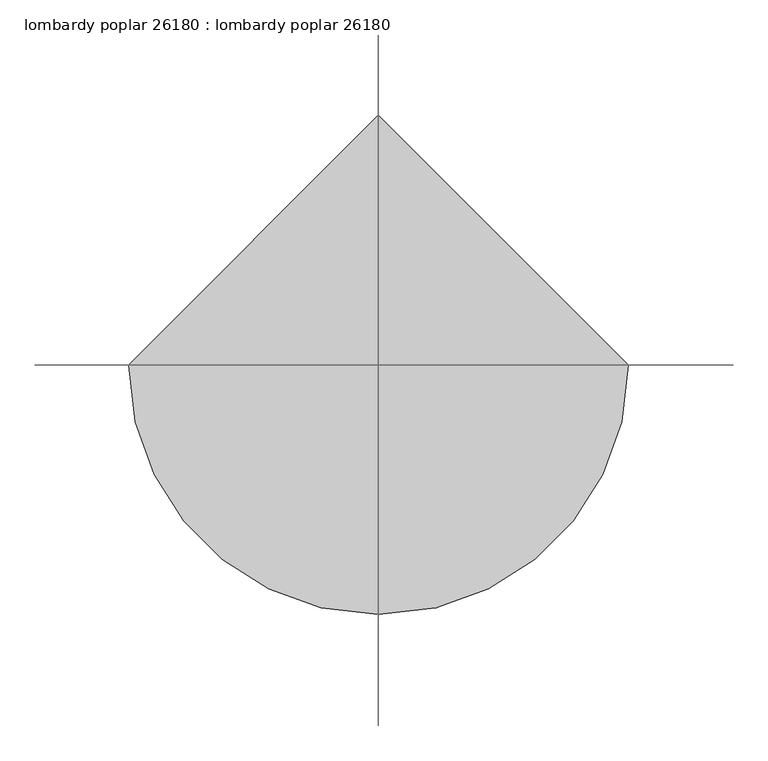
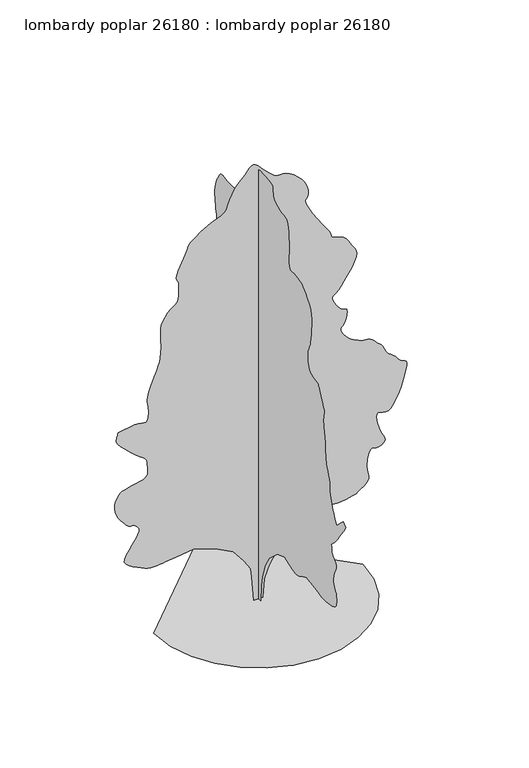
"""IFC4 building model written with IfcOpenShell, lengths in millimetres: proxy geometry, lombardy poplar 26180 : lombardy poplar 26180."""

from ifc_helpers import new_model, si_unit, origin, place, context, project, spatial, triangles, source, transform, mapped, element, save


def lombardy_poplar_26180_lombardy_poplar_26180_01077960(model_context):
    return source(origin(), model_context, "Body", "Tessellation", [
        triangles([(0.0009695, 113.8156909, 0.0), (0.0009695, -104.8345258, 0.0), (0.0009695, -123.055434, 437.3009239), (0.0009695, -177.7179314, 728.8340738), (0.0009695, -323.483707, 1129.6911467), (0.0009695, -505.6928613, 1439.4461494), (0.0009695, -870.1086628, 1767.420607), (0.0009695, -1216.3049732, 1894.9664555), (0.0009695, -1398.5142002, 1822.0838402), (0.0009695, -1476.390406, 1795.1523445), (0.0009695, -1552.9941605, 1770.6083485), (0.0009695, -1627.0451637, 1750.8472), (0.0009695, -1697.2735806, 1738.2588696), (0.0009695, -1762.3991112, 1735.2286766), (0.0009695, -1821.1516296, 1744.1542946), (0.0009695, -1872.2563591, 1767.420607), (0.0009695, -1919.1091679, 1797.0624023), (0.0009695, -1965.9644474, 1823.8364948), (0.0009695, -2012.8172562, 1848.2204716), (0.0009695, -2059.6700649, 1870.6891582), (0.0009695, -2106.5227283, 1891.7279903), (0.0009695, -2153.3780079, 1911.8067066), (0.0009695, -2200.2308167, 1931.4103065), (0.0009695, -2582.8711235, 1876.7470734), (0.0009695, -2649.2156204, 1861.2353748), (0.0009695, -2715.4080917, 1846.3611374), (0.0009695, -2781.27006, 1832.7619675), (0.0009695, -2846.6750793, 1821.0754715), (0.0009695, -2911.4196739, 1811.9366398), (0.0009695, -2975.3765259, 1805.987875), (0.0009695, -3038.3939003, 1803.8619873), (0.0009695, -3111.6472778, 1806.252103), (0.0009695, -3200.5217949, 1814.0625275), (0.0009695, -3296.0764275, 1828.2459641), (0.0009695, -3389.4213112, 1849.7596218), (0.0009695, -3471.5901329, 1879.5614365), (0.0009695, -3533.6930283, 1918.6062916), (0.0009695, -3566.7892639, 1967.8516869), (0.0009695, -3579.2353065, 2021.4507408), (0.0009695, -3585.9154221, 2073.1371208), (0.0009695, -3587.8205383, 2123.2333363), (0.0009695, -3585.9154221, 2172.0521587), (0.0009695, -3581.1401321, 2219.915807), (0.0009695, -3574.4347275, 2267.139378), (0.0009695, -3566.7892639, 2314.0455265), (0.0009695, -3532.0422569, 2353.5170998), (0.0009695, -3499.7078934, 2395.5361919), (0.0009695, -3472.1235306, 2442.6555542), (0.0009695, -3451.7273918, 2497.4231415), (0.0009695, -3440.907122, 2562.3988266), (0.0009695, -3441.9992065, 2640.0972816), (0.0009695, -3457.4677391, 2733.1372421), (0.0009695, -3484.5187042, 2825.1865654), (0.0009695, -3515.3799019, 2900.6752716), (0.0009695, -3544.9708282, 2963.0830902), (0.0009695, -3568.1862717, 3015.940329), (0.0009695, -3579.9210205, 3062.7525879), (0.0009695, -3575.0695724, 3106.9993057), (0.0009695, -3548.5775848, 3152.2110809), (0.0009695, -3509.7918709, 3193.1050964), (0.0009695, -3472.6063499, 3225.0836678), (0.0009695, -3438.6212151, 3252.6171616), (0.0009695, -3409.3857903, 3280.1253662), (0.0009695, -3386.5511375, 3312.1039375), (0.0009695, -3371.6668716, 3352.997953), (0.0009695, -3366.3581841, 3407.3030685), (0.0009695, -3362.7005585, 3460.5158089), (0.0009695, -3354.9027786, 3498.4634926), (0.0009695, -3347.7145546, 3525.8699593), (0.0009695, -3345.9620453, 3547.5360786), (0.0009695, -3354.4202499, 3568.2624298), (0.0009695, -3377.8388786, 3592.7987228), (0.0009695, -3421.0188011, 3625.9458275), (0.0009695, -3481.5215034, 3679.8698616), (0.0009695, -3552.5654228, 3760.5655174), (0.0009695, -3632.3465996, 3863.5624283), (0.0009695, -3719.1381042, 3984.4155167), (0.0009695, -3811.2130074, 4118.6541252), (0.0009695, -3906.7676399, 4261.8084686), (0.0009695, -4004.1003616, 4409.432888), (0.0009695, -3894.7788368, 4518.779702), (0.0009695, -3749.0086647, 4391.221209), (0.0009695, -3603.2382019, 4227.2390671), (0.0009695, -3579.7434151, 4258.785688), (0.0009695, -3555.9689941, 4292.2630051), (0.0009695, -3531.5088593, 4329.5499733), (0.0009695, -3506.1342453, 4372.5775795), (0.0009695, -3479.4643616, 4423.2506493), (0.0009695, -3451.1939941, 4483.4992973), (0.0009695, -3421.0188011, 4555.2033508), (0.0009695, -3390.0055779, 4628.5837555), (0.0009695, -3360.2623352, 4695.8683113), (0.0009695, -3333.0587631, 4762.2383881), (0.0009695, -3309.6910034, 4832.7233299), (0.0009695, -3291.4028755, 4912.4536377), (0.0009695, -3279.5158104, 5006.5351044), (0.0009695, -3275.248629, 5120.0473618), (0.0009695, -3267.0697678, 5234.8554703), (0.0009695, -3245.5050957, 5333.3820145), (0.0009695, -3215.0252701, 5421.7481323), (0.0009695, -3180.0747871, 5505.9238083), (0.0009695, -3145.0993057, 5592.0551788), (0.0009695, -3114.6191895, 5686.1110657), (0.0009695, -3093.0545174, 5794.238768), (0.0009695, -3079.5672592, 5892.1298859), (0.0009695, -3069.8899429, 5959.4403122), (0.0009695, -3063.4130127, 6007.9286316), (0.0009695, -3059.4760437, 6049.4319122), (0.0009695, -3057.4691895, 6095.6854843), (0.0009695, -3056.7073174, 6158.5246719), (0.0009695, -3056.6055794, 6249.735965), (0.0009695, -3052.5671631, 6343.1320084), (0.0009695, -3042.1532639, 6412.2958099), (0.0009695, -3027.9291321, 6468.709227), (0.0009695, -3012.4097305, 6523.8523727), (0.0009695, -2998.1858894, 6589.2065231), (0.0009695, -2987.7716995, 6676.2017944), (0.0009695, -2983.7332832, 6796.3688782), (0.0009695, -2989.2957344, 6908.7381821), (0.0009695, -3001.5638809, 6976.78461), (0.0009695, -3013.8576073, 7018.6948425), (0.0009695, -3019.4200584, 7052.6288177), (0.0009695, -3011.6222786, 7096.7737976), (0.0009695, -2983.7332832, 7169.2908829), (0.0009695, -2929.0723755, 7288.340593), (0.0009695, -2866.7410057, 7418.1088348), (0.0009695, -2818.7857933, 7514.4256302), (0.0009695, -2782.7688057, 7582.8528488), (0.0009695, -2756.3021072, 7628.9541046), (0.0009695, -2737.0233421, 7658.3418457), (0.0009695, -2722.5201576, 7676.5535248), (0.0009695, -2710.4043274, 7689.2027527), (0.0009695, -2636.5666832, 7701.2421341), (0.0009695, -2564.8117607, 7715.3901077), (0.0009695, -2497.1818771, 7733.6523651), (0.0009695, -2435.7748695, 7758.1380798), (0.0009695, -2382.6507866, 7790.9296829), (0.0009695, -2339.8900246, 7834.0584457), (0.0009695, -2309.5548122, 7889.6335419), (0.0009695, -2289.3160767, 7951.0257248), (0.0009695, -2274.8152176, 8010.5377899), (0.0009695, -2265.0921192, 8068.4243729), (0.0009695, -2259.1968395, 8125.0662643), (0.0009695, -2256.1691174, 8180.7425171), (0.0009695, -2255.0515984, 8235.7589264), (0.0009695, -2254.8940498, 8290.4707031), (0.0009695, -2285.970932, 8345.7405853), (0.0009695, -2316.0901691, 8404.491069), (0.0009695, -2344.2968777, 8470.25159), (0.0009695, -2369.6358833, 8546.5277481), (0.0009695, -2391.1521572, 8636.8495605), (0.0009695, -2407.8857288, 8744.6726303), (0.0009695, -2418.8812786, 8873.551973), (0.0009695, -2430.0903328, 9004.9206985), (0.0009695, -2443.8493767, 9121.3031296), (0.0009695, -2453.7833633, 9227.8303482), (0.0009695, -2453.5168098, 9329.5572784), (0.0009695, -2436.6765587, 9431.5888412), (0.0009695, -2396.8874176, 9539.0561188), (0.0009695, -2327.7766651, 9657.0390335), (0.0009695, -2247.8811058, 9768.2398041), (0.0009695, -2177.228587, 9854.8798645), (0.0009695, -2111.6764835, 9921.4269653), (0.0009695, -2047.0792637, 9972.3796692), (0.0009695, -1979.2969185, 10012.156311), (0.0009695, -1904.1815907, 10045.2519653), (0.0009695, -1817.5931259, 10076.1128723), (0.0009695, -1725.5334835, 10094.8326599), (0.0009695, -1638.891679, 10096.3058258), (0.0009695, -1560.8554539, 10092.3688568), (0.0009695, -1494.6124043, 10094.8326599), (0.0009695, -1443.3501263, 10115.4325653), (0.0009695, -1410.2540359, 10166.0038971), (0.0009695, -1398.5142002, 10258.3319824), (0.0009695, -1400.4267288, 10362.6756134), (0.0009695, -1404.8895378, 10448.1971375), (0.0009695, -1409.9898079, 10525.1087219), (0.0009695, -1413.8125397, 10603.619046), (0.0009695, -1414.4501461, 10693.9414398), (0.0009695, -1409.9898079, 10806.2345856), (0.0009695, -1398.5142002, 10950.7350677), (0.0009695, -1382.6849339, 11097.4458801), (0.0009695, -1365.5779839, 11211.9737732), (0.0009695, -1345.9235149, 11297.8255096), (0.0009695, -1322.4438435, 11358.4811096), (0.0009695, -1293.8637566, 11397.4694275), (0.0009695, -1258.9083321, 11418.297226), (0.0009695, -1216.3049732, 11424.470105), (0.0009695, -1155.4822323, 11429.9813965), (0.0009695, -1073.3006933, 11446.3641174), (0.0009695, -979.6484882, 11473.2380585), (0.0009695, -884.3986336, 11510.3218414), (0.0009695, -797.4393339, 11557.2608368), (0.0009695, -728.6460766, 11613.8015717), (0.0009695, -687.9020519, 11679.5615112), (0.0009695, -672.8677952, 11749.3607391), (0.0009695, -668.0341513, 11816.289212), (0.0009695, -663.5180752, 11877.4785004), (0.0009695, -649.4413908, 11930.0811035), (0.0009695, -615.9210531, 11971.2041748), (0.0009695, -553.0790314, 11997.9757965), (0.0009695, -451.0296281, 12007.5263763), (0.0009695, -327.7864603, 12011.2087097), (0.0009695, -210.2816959, 12019.0070709), (0.0009695, -102.0189364, 12026.1694244), (0.0009695, -6.5056406, 12027.9216431), (0.0009695, 72.7523407, 12019.4895996), (0.0009695, 132.2489498, 11996.0700989), (0.0009695, 168.4781792, 11952.8657593), (0.0009695, 190.2581361, 11903.7920105), (0.0009695, 211.0820467, 11861.400412), (0.0009695, 234.4553475, 11819.0076508), (0.0009695, 263.8852554, 11769.9094849), (0.0009695, 302.8767344, 11707.4505066), (0.0009695, 354.9364746, 11624.9008942), (0.0009695, 423.5697126, 11515.57966), (0.0009695, 499.5867296, 11399.1204895), (0.0009695, 572.09851, 11297.9778259), (0.0009695, 642.0601553, 11209.5867096), (0.0009695, 710.4292379, 11131.3798553), (0.0009695, 778.1582434, 11060.8446259), (0.0009695, 846.2072874, 10995.3881561), (0.0009695, 915.531399, 10932.4978088), (0.0009695, 983.7404623, 10880.5556305), (0.0009695, 1048.444289, 10847.0786041), (0.0009695, 1110.5954372, 10828.282077), (0.0009695, 1171.1565662, 10820.3069824), (0.0009695, 1231.077618, 10819.3407623), (0.0009695, 1291.3160923, 10821.5766724), (0.0009695, 1352.8322502, 10823.1765747), (0.0009695, 1419.1287849, 10828.7646057), (0.0009695, 1490.5254444, 10841.0324615), (0.0009695, 1563.194846, 10853.3014801), (0.0009695, 1633.3164379, 10858.8639313), (0.0009695, 1697.0626923, 10851.0655701), (0.0009695, 1750.6084064, 10823.1765747), (0.0009695, 1790.1333195, 10768.5159576), (0.0009695, 1824.1844387, 10700.9526398), (0.0009695, 1861.7408672, 10636.2333344), (0.0009695, 1899.617189, 10570.5745514), (0.0009695, 1934.6234825, 10500.1404785), (0.0009695, 1963.5743317, 10421.0953033), (0.0009695, 1983.2847565, 10329.6299561), (0.0009695, 1990.5617832, 10221.8830444), (0.0009695, 1988.4357502, 10111.0130676), (0.0009695, 1982.4871307, 10010.9877777), (0.0009695, 1973.3507698, 9919.2433777), (0.0009695, 1961.6642738, 9833.2381622), (0.0009695, 1948.0651039, 9750.4350769), (0.0009695, 1933.1908665, 9668.2656738), (0.0009695, 1917.6791679, 9584.1667374), (0.0009695, 1914.3314072, 9505.3761978), (0.0009695, 1931.0649788, 9438.0663528), (0.0009695, 1961.1842159, 9378.0967575), (0.0009695, 1997.9989746, 9321.3025497), (0.0009695, 2034.813588, 9263.5682831), (0.0009695, 2064.9328251, 9200.7290955), (0.0009695, 2081.6663967, 9128.6439606), (0.0009695, 2081.1888096, 9058.6668365), (0.0009695, 2066.6854797, 9001.7964706), (0.0009695, 2041.9840805, 8953.1808334), (0.0009695, 2010.9071983, 8908.0707962), (0.0009695, 1977.2826519, 8861.6904877), (0.0009695, 1944.9307022, 8809.2646179), (0.0009695, 1917.6791679, 8745.9934799), (0.0009695, 1901.8472855, 8673.7048691), (0.0009695, 1900.361475, 8598.2164536), (0.0009695, 1911.9412914, 8520.8229218), (0.0009695, 1935.3142834, 8442.7939636), (0.0009695, 1969.2055286, 8365.374852), (0.0009695, 2012.3422852, 8289.8864365), (0.0009695, 2063.4443985, 8217.5978256), (0.0009695, 2116.1951031, 8158.060762), (0.0009695, 2166.3955273, 8113.7884644), (0.0009695, 2215.9584904, 8075.6123062), (0.0009695, 2266.796521, 8034.2101822), (0.0009695, 2320.8222931, 7980.4134659), (0.0009695, 2379.9457191, 7904.924469), (0.0009695, 2446.0820892, 7798.5239868), (0.0009695, 2515.4595406, 7684.1478287), (0.0009695, 2583.8870499, 7588.5931961), (0.0009695, 2652.6194824, 7508.3039108), (0.0009695, 2722.9518173, 7439.8511124), (0.0009695, 2796.1546165, 7379.653624), (0.0009695, 2873.4972794, 7324.2558426), (0.0009695, 2956.2759476, 7270.103334), (0.0009695, 3039.9940933, 7227.3042023), (0.0009695, 3119.5720848, 7202.0063278), (0.0009695, 3195.3148453, 7185.0137604), (0.0009695, 3267.5522964, 7167.0555542), (0.0009695, 3336.6149414, 7138.9125046), (0.0009695, 3402.807122, 7091.3130844), (0.0009695, 3466.4593414, 7015.0113464), (0.0009695, 3525.2604034, 6921.5903046), (0.0009695, 3575.4506538, 6829.7441666), (0.0009695, 3615.1508469, 6741.0728348), (0.0009695, 3642.3797081, 6657.2023727), (0.0009695, 3655.3082794, 6579.6815231), (0.0009695, 3651.9552864, 6510.1619293), (0.0009695, 3630.4414833, 6450.1673355), (0.0009695, 3590.004998, 6392.5348068), (0.0009695, 3534.6075073, 6330.4316208), (0.0009695, 3469.3295151, 6266.1192673), (0.0009695, 3399.2512344, 6201.7813339), (0.0009695, 3329.5028755, 6139.6781479), (0.0009695, 3265.1646515, 6082.0456192), (0.0009695, 3211.3676445, 6031.0934967), (0.0009695, 3161.7869499, 5985.0939789), (0.0009695, 3109.3613708, 5939.7298874), (0.0009695, 3057.8758507, 5893.4001572), (0.0009695, 3011.1906189, 5844.5304657), (0.0009695, 2973.1159081, 5791.5209106), (0.0009695, 2947.4366615, 5732.7710083), (0.0009695, 2938.0386887, 5666.680275), (0.0009695, 2934.1778778, 5597.4141541), (0.0009695, 2924.8816429, 5529.7235184), (0.0009695, 2913.6547119, 5463.0235199), (0.0009695, 2904.0535538, 5396.6025742), (0.0009695, 2899.5323181, 5329.8764145), (0.0009695, 2903.6218941, 5262.2113586), (0.0009695, 2919.8270096, 5192.9452377), (0.0009695, 2944.8458313, 5126.3719757), (0.0009695, 2972.7351173, 5066.5046997), (0.0009695, 3003.0117577, 5012.2248734), (0.0009695, 3035.1935143, 4962.3901245), (0.0009695, 3068.8231476, 4915.908078), (0.0009695, 3103.4178383, 4871.6613602), (0.0009695, 3138.4697685, 4828.5323067), (0.0009695, 3181.1415825, 4835.3141602), (0.0009695, 3222.035598, 4836.0760323), (0.0009695, 3259.4243042, 4824.696785), (0.0009695, 3291.5807716, 4795.1567276), (0.0009695, 3316.7013313, 4741.4102989), (0.0009695, 3333.0587631, 4657.3619408), (0.0009695, 3338.9008484, 4536.9916718), (0.0009695, 3338.9008484, 3935.6984322), (0.0009695, 3345.6065437, 3757.6444748), (0.0009695, 3361.2273926, 3611.1377197), (0.0009695, 3379.0582809, 3492.0371407), (0.0009695, 3392.4440918, 3396.2031647), (0.0009695, 3394.6791298, 3319.4953468), (0.0009695, 3379.0582809, 3257.747953), (0.0009695, 3338.9008484, 3206.8719887), (0.0009695, 3281.573243, 3178.2461197), (0.0009695, 3221.7053856, 3174.1568344), (0.0009695, 3163.4380119, 3176.747374), (0.0009695, 3110.9106949, 3168.187722), (0.0009695, 3068.2388809, 3130.6466995), (0.0009695, 3039.6130119, 3046.21726), (0.0009695, 3029.1482437, 2897.119384), (0.0009695, 3036.0571243, 2732.8070297), (0.0009695, 3053.1514297, 2608.9823204), (0.0009695, 3075.0460236, 2517.0268867), (0.0009695, 3096.3057724, 2448.3400909), (0.0009695, 3111.4949615, 2394.3144642), (0.0009695, 3115.2034561, 2346.3441364), (0.0009695, 3102.0208305, 2295.8261444), (0.0009695, 3089.0669701, 2254.1778145), (0.0009695, 3089.803553, 2232.6106716), (0.0009695, 3093.4355988, 2222.1992432), (0.0009695, 3089.0669701, 2214.0179111), (0.0009695, 3065.9021049, 2199.1436737), (0.0009695, 3013.0954445, 2168.6510582), (0.0009695, 2919.8270096, 2113.6169174), (0.0009695, 2822.3419716, 2052.8450455), (0.0009695, 2753.55867, 2008.9666191), (0.0009695, 2697.5010452, 1978.7940422), (0.0009695, 2638.2683235, 1959.1395733), (0.0009695, 2559.9350235, 1946.8154709), (0.0009695, 2446.5088074, 1938.6341389), (0.0009695, 2282.0948605, 1931.4103065), (0.0009695, 2105.8903542, 1933.6938881), (0.0009695, 1963.4702682, 1951.9132702), (0.0009695, 1848.4591198, 1979.6982021), (0.0009695, 1754.4869488, 2010.665934), (0.0009695, 1675.1755108, 2038.4483952), (0.0009695, 1604.1522297, 2056.670248), (0.0009695, 1535.0414772, 2058.9536842), (0.0009695, 1460.510416, 2049.0198429), (0.0009695, 1378.3312752, 2035.2631245), (0.0009695, 1289.7769421, 2018.3163391), (0.0009695, 1196.1221935, 1998.8218895), (0.0009695, 1098.6447859, 1977.4122952), (0.0009695, 998.6146271, 1954.7301041), (0.0009695, 897.3120169, 1931.4103065), (0.0009695, 532.8936719, 1639.8747585), (0.0009695, 314.2457534, 1166.1349977), (0.0009695, 168.4781792, 601.2881527), (120.1776209, 0.0005334, 0.0085345), (-116.69275, 0.0005334, 0.0085345), (-171.3552383, 0.0004849, 655.9590162), (-207.7973272, 0.0004849, 911.0508585), (-390.006209, 0.0004607, 1202.5839357), (-663.3174334, 0.0004364, 1548.7803188), (-1137.0596649, 0.0004122, 1803.8721611), (-1720.1284355, 0.0004122, 1986.078772), (-2193.8681236, 0.0004122, 1931.4180096), (-2467.1819641, 0.0004122, 1894.9766293), (-2533.7959213, 0.0004122, 1885.46689), (-2607.4327057, 0.0004122, 1874.6820831), (-2686.1473778, 0.0004122, 1865.812421), (-2768.0621452, 0.0004122, 1862.0405582), (-2851.2468933, 0.0004122, 1866.556707), (-2933.7967964, 0.0004122, 1882.5459927), (-3013.8067383, 0.0004122, 1913.1960114), (-3104.2814484, 0.0004122, 1955.5886272), (-3210.9865631, 0.0004122, 2004.6715324), (-3321.222567, 0.0004122, 2060.4522846), (-3422.2126236, 0.0004122, 2122.9234715), (-3501.2066391, 0.0003879, 2192.0875637), (-3545.4533569, 0.0003879, 2267.9445614), (-3542.2021019, 0.0003879, 2350.4969353), (-3495.1869484, 0.0003879, 2447.2326004), (-3424.930481, 0.0003879, 2559.9094437), (-3343.8031654, 0.0003637, 2679.898922), (-3264.2757523, 0.0003637, 2798.6437088), (-3198.7692856, 0.0003637, 2907.4824142), (-3159.7295174, 0.0003394, 2997.8300972), (-3159.5772011, 0.0003394, 3061.1015259), (-3182.9958298, 0.0003394, 3103.1893639), (-3206.4147491, 0.0003394, 3136.6411011), (-3229.8589577, 0.0003394, 3162.9554832), (-3253.2775864, 0.0003394, 3183.5039383), (-3276.6962151, 0.0003394, 3199.7599228), (-3300.1404236, 0.0003394, 3213.1457336), (-3323.559343, 0.0003394, 3225.1089569), (-3347.1558678, 0.0003394, 3221.5783585), (-3371.6921608, 0.0003394, 3220.486274), (-3398.1335701, 0.0003394, 3224.1438995), (-3427.4704422, 0.0003394, 3234.9897491), (-3460.6175468, 0.0003394, 3255.3858879), (-3498.5396507, 0.0003394, 3287.7199608), (-3542.2021019, 0.0003394, 3334.4304817), (-3593.6370438, 0.0003394, 3395.5174507), (-3650.1519081, 0.0003152, 3468.3897469), (-3705.7270042, 0.0003152, 3551.4730476), (-3754.2664833, 0.0003152, 3643.1668694), (-3789.7500732, 0.0003152, 3741.8713097), (-3806.1330849, 0.0002909, 3845.9855942), (-3797.2937988, 0.0002909, 3953.9354004), (-3771.4366562, 0.0002909, 4051.5730453), (-3739.8138771, 0.0002909, 4128.1791252), (-3701.2057686, 0.0002909, 4187.2342415), (-3654.2920624, 0.0002667, 4232.2937004), (-3597.828067, 0.0002667, 4266.812233), (-3530.518222, 0.0002667, 4294.3457268), (-3451.117836, 0.0002667, 4318.3486221), (-3356.8078949, 0.0002667, 4338.3131012), (-3252.3378181, 0.0002667, 4355.4326958), (-3147.5122398, 0.0002667, 4375.7270966), (-3052.2622398, 0.0002667, 4405.2674446), (-2976.4689011, 0.0002667, 4450.0981384), (-2929.9868546, 0.0002667, 4516.2906097), (-2922.6971832, 0.0002667, 4609.8895477), (-2933.5936111, 0.0002425, 4707.6283493), (-2938.4197701, 0.0002425, 4784.9713028), (-2942.3058701, 0.0002425, 4846.0582718), (-2950.332415, 0.0002425, 4895.0291199), (-2967.578746, 0.0002425, 4936.0504532), (-2999.2018158, 0.0002425, 4973.2359741), (-3050.2556763, 0.0002425, 5010.7517075), (-3135.4978569, 0.0002182, 5072.041571), (-3254.8777794, 0.0002182, 5168.7141586), (-3391.1232422, 0.0002182, 5287.0778641), (-3527.0637817, 0.0002182, 5413.3916656), (-3645.4783562, 0.000194, 5533.9906998), (-3729.1459236, 0.000194, 5635.1333633), (-3760.8704407, 0.000194, 5703.129213), (-3759.2702477, 0.000194, 5747.3247711), (-3754.799881, 0.000194, 5786.7456207), (-3747.9418694, 0.000194, 5822.178923), (-3739.1787415, 0.0001697, 5854.4112579), (-3728.9933167, 0.0001697, 5884.2815277), (-3717.8428345, 0.0001697, 5912.5263153), (-3706.2095329, 0.0001697, 5940.0089401), (-3268.8984352, 0.0001697, 6012.8818176), (-3174.1312546, 0.0001697, 6014.48172), (-3093.0545174, 0.0001697, 5998.8605804), (-3026.0240158, 0.0001697, 5982.2743835), (-2973.319384, 0.0001697, 5981.0046936), (-2935.2955421, 0.0001697, 6011.2813339), (-2912.232415, 0.0001697, 6089.3864502), (-2904.4852135, 0.0001697, 6231.5242859), (-2910.9624344, 0.0001455, 6377.1421417), (-2925.0848282, 0.0001455, 6470.4870255), (-2938.9022987, 0.0001455, 6535.1301727), (-2944.4394608, 0.0001455, 6594.6678177), (-2933.6953491, 0.0001212, 6672.7217743), (-2898.7448662, 0.0001212, 6792.8126999), (-2831.5873375, 0.0001212, 6978.5879883), (-2754.346122, 9.7e-05, 7175.5649185), (-2693.3861801, 9.7e-05, 7325.0435852), (-2647.0567406, 9.7e-05, 7444.2456116), (-2613.8081886, 7.27e-05, 7550.3920395), (-2592.0150421, 7.27e-05, 7660.678331), (-2580.127977, 7.27e-05, 7792.3011108), (-2576.4956406, 4.85e-05, 7962.5064194), (-2580.0009499, 4.85e-05, 8135.9626923), (-2586.7063545, 4.85e-05, 8272.4363388), (-2590.8467995, 2.42e-05, 8381.8087326), (-2586.7063545, 2.42e-05, 8473.985083), (-2568.5455444, 2.42e-05, 8558.8211838), (-2530.6106506, 2.42e-05, 8646.1972458), (-2467.1819641, 0.0, 8746.0190598), (-2393.5550629, 0.0, 8838.8046753), (-2328.8511635, 0.0, 8903.8797729), (-2273.0728821, 0.0, 8949.1932861), (-2226.2200733, 0.0, 8982.7208908), (-2188.2902664, 0.0, 9012.4138458), (-2159.2860775, 0.0, 9046.2460831), (-2139.2048904, 0.0, 9092.1950226), (-2125.7124001, -2.42e-05, 9135.3493652), (-2116.0452576, -2.42e-05, 9162.8575699), (-2109.5630951, -2.42e-05, 9185.920697), (-2105.6338291, -2.42e-05, 9215.6642303), (-2103.6144756, -2.42e-05, 9263.2636505), (-2102.8701897, -2.42e-05, 9339.8700211), (-2102.7661263, -2.42e-05, 9456.6332428), (-2113.0708752, -4.85e-05, 9567.5549606), (-2136.1264446, -4.85e-05, 9634.4840149), (-2160.137043, -4.85e-05, 9680.3817947), (-2173.3094948, -4.85e-05, 9728.1846909), (-2163.855566, -4.85e-05, 9800.8540924), (-2119.9745235, -7.27e-05, 9921.3258087), (-2029.8808949, -7.27e-05, 10112.5618103), (-1939.4672276, -7.27e-05, 10305.830246), (-1888.8958958, -9.7e-05, 10431.5097839), (-1857.7656738, -9.7e-05, 10511.3165405), (-1825.6805683, -9.7e-05, 10566.8654755), (-1772.2389175, -9.7e-05, 10619.9006104), (-1677.0450188, -9.7e-05, 10692.0369049), (-1519.6973557, -0.0001212, 10804.9648956), (-1341.6868549, -0.0001212, 10917.309201), (-1195.5481733, -0.0001212, 10985.3806274), (-1077.4586517, -0.0001212, 11027.29086), (-983.5905441, -0.0001212, 11061.2248352), (-910.1237349, -0.0001212, 11105.3698151), (-853.2303326, -0.0001455, 11177.8874817), (-809.0852074, -0.0001455, 11296.9371918), (-759.9464916, -0.0001455, 11440.4714539), (-694.8717573, -0.0001697, 11572.8563965), (-620.2365601, -0.0001697, 11691.8293671), (-542.413585, -0.0001697, 11795.2079407), (-467.775808, -0.0001697, 11880.7294647), (-402.7036534, -0.0001697, 11946.1847717), (-353.5649014, -0.000194, 11989.3146973), (-315.2642959, -0.000194, 12029.8529205), (-276.9611651, -0.000194, 12081.541626), (-236.4299363, -0.000194, 12133.2303314), (-191.4351718, -0.000194, 12173.7685547), (-139.7475292, -0.000194, 12191.9802338), (-79.1353495, -0.000194, 12176.7404663), (-7.3676139, -0.000194, 12116.8731903), (68.4904824, -0.000194, 12035.3130524), (139.8862108, -0.000194, 11962.0605469), (206.8199341, -0.0001697, 11896.4517609), (269.290376, -0.0001697, 11837.8797546), (327.3013518, -0.0001697, 11785.6573608), (380.8469934, -0.0001697, 11739.1753143), (429.9324057, -0.0001697, 11697.7987701), (477.3160323, -0.0001697, 11672.4491547), (527.8899076, -0.0001697, 11666.8622864), (584.8366133, -0.0001697, 11669.5795624), (651.343891, -0.0001697, 11669.0970337), (730.6019165, -0.0001697, 11653.9584229), (825.7958879, -0.0001697, 11612.684198), (940.1160175, -0.0001455, 11533.7913391), (1053.1051964, -0.0001455, 11434.3508972), (1143.4680674, -0.0001455, 11338.4148926), (1213.1096741, -0.0001455, 11245.0194305), (1263.9477047, -0.0001455, 11153.2238708), (1297.8921444, -0.0001212, 11062.0631561), (1316.8558125, -0.0001212, 10970.5978088), (1322.7537083, -0.0001212, 10877.8371918), (1310.6404942, -0.0001212, 10807.3019623), (1283.8688725, -0.0001212, 10768.6426941), (1256.7747414, -0.0001212, 10740.1444336), (1243.7064983, -9.7e-05, 10700.2154755), (1259.0074539, -9.7e-05, 10627.1141235), (1317.0158318, -9.7e-05, 10499.1998383), (1432.0777039, -7.27e-05, 10294.7809204), (1568.3356659, -7.27e-05, 10074.4362305), (1681.0074223, -4.85e-05, 9906.365094), (1771.0503273, -4.85e-05, 9780.3565063), (1839.4167938, -4.85e-05, 9686.22388), (1887.067083, -4.85e-05, 9613.757373), (1914.9562237, -4.85e-05, 9552.772142), (1924.041861, -2.42e-05, 9493.0571823), (1943.5896503, -2.42e-05, 9444.2892288), (1995.6494087, -2.42e-05, 9415.2822784), (2070.3380184, -2.42e-05, 9394.5812164), (2157.7773033, -2.42e-05, 9370.6797684), (2248.0842911, -2.42e-05, 9332.0972397), (2331.3809509, -2.42e-05, 9267.4035141), (2397.7841652, -2.42e-05, 9165.0928986), (2454.6240097, 0.0, 9055.2379761), (2511.1467224, 0.0, 8968.9542892), (2560.341394, 0.0, 8896.3866257), (2595.190139, 0.0, 8827.6541931), (2608.6773972, 0.0, 8752.8512009), (2593.7931313, 2.42e-05, 8662.1230179), (2543.5520119, 2.42e-05, 8545.5876892), (2481.3447624, 2.42e-05, 8432.1260101), (2431.8886242, 2.42e-05, 8349.5508179), (2390.080275, 2.42e-05, 8286.457576), (2350.8220608, 4.85e-05, 8231.3138489), (2309.0163277, 4.85e-05, 8172.6656845), (2259.5600441, 4.85e-05, 8099.0312256), (2197.3530853, 4.85e-05, 7998.9553574), (2127.0206051, 4.85e-05, 7904.0355698), (2060.8307499, 7.27e-05, 7844.1677124), (2005.159148, 7.27e-05, 7805.3311295), (1966.378521, 7.27e-05, 7773.5051651), (1950.8666771, 7.27e-05, 7734.6685822), (1964.9992447, 7.27e-05, 7674.8007248), (2015.1464745, 7.27e-05, 7579.8815186), (2080.6452381, 7.27e-05, 7478.1545883), (2137.5387131, 9.7e-05, 7404.1387573), (2187.2590794, 9.7e-05, 7353.262793), (2231.2468014, 9.7e-05, 7320.852562), (2270.9265015, 9.7e-05, 7302.3106705), (2307.7412601, 9.7e-05, 7293.0141449), (2343.1207867, 9.7e-05, 7288.340593), (2346.839455, 9.7e-05, 7260.6544922), (2349.4429298, 9.7e-05, 7230.9109589), (2349.8136921, 9.7e-05, 7197.027562), (2346.839455, 9.7e-05, 7156.9212891), (2339.4022636, 9.7e-05, 7108.5341263), (2326.3873604, 0.0001212, 7049.7842239), (2306.6795517, 0.0001212, 6978.5879883), (2277.832766, 0.0001212, 6914.427951), (2243.2507198, 0.0001212, 6871.273027), (2210.5813477, 0.0001212, 6838.9901138), (2187.4724384, 0.0001212, 6807.3158844), (2181.5771587, 0.0001212, 6766.0922379), (2200.5406815, 0.0001212, 6705.1064255), (2252.0163185, 0.0001455, 6614.1747665), (2322.1379105, 0.0001455, 6519.5090332), (2391.3020027, 0.0001455, 6450.3452316), (2458.553421, 0.0001455, 6400.9424332), (2522.9372818, 0.0001455, 6365.5602905), (2583.5059685, 0.0001455, 6338.4584564), (2639.2842499, 0.0001455, 6313.9221634), (2689.322184, 0.0001455, 6286.184903), (2738.2427444, 0.0001455, 6263.7822006), (2790.6680328, 0.0001455, 6254.1048843), (2845.659153, 0.0001697, 6249.8632828), (2902.2248863, 0.0001697, 6243.6909851), (2959.4507538, 0.0001697, 6228.2989014), (3016.3466995, 0.0001697, 6196.3200394), (3071.9473755, 0.0001697, 6140.4403107), (3121.4519119, 0.0001697, 6084.0774719), (3162.3712166, 0.0001697, 6048.746489), (3197.2199615, 0.0001697, 6024.2607742), (3228.5633972, 0.0001697, 6000.4104858), (3258.9417755, 0.0001697, 5966.9840378), (3290.9203468, 0.0001697, 5913.8215851), (3327.0390724, 0.000194, 5830.687706), (3367.3235321, 0.000194, 5746.3091354), (3410.4525856, 0.000194, 5689.0573975), (3457.0869484, 0.000194, 5648.0366455), (3507.8614655, 0.000194, 5612.4510269), (3563.4365616, 0.000194, 5571.430275), (3624.4217926, 0.000194, 5514.178537), (3691.4522942, 0.0002182, 5429.8255463), (3759.9306725, 0.0002182, 5354.920816), (3822.0335678, 0.0002182, 5319.208461), (3873.620826, 0.0002182, 5301.6827866), (3910.5270035, 0.0002182, 5281.2863571), (3928.6625244, 0.0002182, 5236.989061), (3923.8110764, 0.0002182, 5147.7334625), (3891.883374, 0.0002425, 4992.5144485), (3839.8897453, 0.0002425, 4801.4304726), (3779.2600159, 0.0002667, 4621.8274818), (3712.6105957, 0.0002667, 4458.4801849), (3642.4302864, 0.0002667, 4316.1641624), (3571.3104996, 0.0002909, 4199.6799934), (3501.7653259, 0.0002909, 4113.777388), (3436.3605972, 0.0002909, 4063.2569252), (3368.5935127, 0.0002909, 4052.055574), (3295.6956367, 0.0002909, 4067.2956322), (3225.9981468, 0.0002909, 4088.6059593), (3167.7813515, 0.0002909, 4095.5657089), (3129.3258499, 0.0002909, 4067.7781609), (3118.9119507, 0.0002909, 3984.8471764), (3144.8452515, 0.0002909, 3826.3769073), (3196.8388802, 0.0003152, 3648.5264259), (3252.998243, 0.0003152, 3514.6686081), (3304.0521034, 0.0003152, 3415.2278755), (3340.7550957, 0.0003394, 3340.6280685), (3353.8615631, 0.0003394, 3281.3444778), (3334.1764275, 0.0003394, 3227.8015251), (3272.3784554, 0.0003394, 3170.4230507), (3191.911274, 0.0003394, 3134.2534561), (3121.6295174, 0.0003394, 3135.3711205), (3060.5934174, 0.0003394, 3150.839653), (3007.8379166, 0.0003394, 3157.6976646), (2962.4226654, 0.0003394, 3132.9834755), (2923.3828972, 0.0003394, 3053.7862747), (2889.7532639, 0.0003637, 2897.119384), (2876.0881096, 0.0003637, 2719.1165863), (2887.6196732, 0.0003879, 2584.1155243), (2909.3366615, 0.0003879, 2481.6546272), (2926.3039398, 0.0003879, 2401.1749466), (2923.4846352, 0.0003879, 2332.1708736), (2885.9180328, 0.0003879, 2264.1218296), (2798.6437088, 0.0003879, 2186.5098518), (2701.5906212, 0.0004122, 2115.113047), (2635.7792313, 0.0004122, 2068.2602383), (2587.7987297, 0.0004122, 2039.2560493), (2544.2885948, 0.0004122, 2021.4075748), (2491.8603996, 0.0004122, 2008.0191479), (2417.1185955, 0.0004122, 1992.4007698), (2306.6795517, 0.0004122, 1967.8592445), (2182.1079403, 0.0004122, 1946.8763683), (2070.9247559, 0.0004122, 1942.7844669), (1968.6644279, 0.0004122, 1950.1707893), (1870.8670544, 0.0004122, 1963.60994), (1773.0695354, 0.0004122, 1977.6865517), (1670.8093529, 0.0004122, 1986.9829319), (1559.6260231, 0.0004122, 1986.078772), (1454.709026, 0.0004122, 1976.1447853), (1371.7857445, 0.0004122, 1962.3882122), (1307.1885246, 0.0004122, 1945.4412815), (1257.2547993, 0.0004122, 1925.9468319), (1218.3166964, 0.0004122, 1904.5372375), (1186.70896, 0.0004122, 1881.8550465), (1158.7664795, 0.0004122, 1858.5353943), (1158.4464409, 0.0004364, 1761.2688023), (1156.2163445, 0.0004364, 1666.0722874), (1150.1584293, 0.0004364, 1575.0234844), (1138.3677246, 0.0004364, 1490.1876743), (1118.9240713, 0.0004364, 1413.6372597), (1089.9198824, 0.0004607, 1347.4475498), (1049.4399405, 0.0004607, 1293.6884766), (1004.179767, 0.0004607, 1251.6160446), (961.7897673, 0.0004607, 1218.1490467), (921.7874125, 0.0004607, 1191.8550121), (883.7001297, 0.0004607, 1171.2962379), (847.045463, 0.0004607, 1155.0403261), (811.3483686, 0.0004607, 1141.6519718), (776.1287888, 0.0004607, 1129.7013205), (466.3737496, 0.0004607, 1129.7013205), (284.1645772, 0.0004849, 856.3875526), (156.6199641, 0.0005092, 510.1912059), (-2766.0555817, 0.0, 0.0100862), (-2692.9292313, -633.8001217, 0.0100862), (-2484.680024, -1215.8427195, 0.0100862), (-2157.9602863, -1729.4553371, 0.0100862), (-1729.4553371, -2157.9602863, 0.0100862), (-1215.8427195, -2484.680024, 0.0100862), (-633.8001217, -2692.9292313, 0.0100862), (0.0001209, -2766.0555817, 0.0100862), (633.8001217, -2692.9292313, 0.0100862), (1215.8427195, -2484.680024, 0.0100862), (1729.4553371, -2157.9602863, 0.0100862), (2157.9602863, -1729.4553371, 0.0100862), (2484.680024, -1215.8427195, 0.0100862), (2692.9292313, -633.8001217, 0.0100862), (2766.0555817, 0.0002425, 0.0100862), (-0.0003627, 2766.0555817, 0.0100862)], [[1, 2, 3], [388, 1, 3], [388, 3, 4], [387, 388, 4], [387, 4, 5], [80, 81, 82], [79, 80, 82], [79, 82, 83], [78, 79, 83], [77, 78, 83], [387, 5, 6], [386, 387, 6], [76, 77, 83], [386, 6, 7], [359, 360, 361], [359, 361, 362], [385, 386, 7], [75, 76, 83], [75, 83, 84], [75, 84, 85], [74, 75, 85], [73, 74, 85], [73, 85, 86], [72, 73, 86], [72, 86, 87], [358, 359, 362], [358, 362, 363], [72, 87, 88], [131, 132, 133], [71, 72, 88], [130, 131, 133], [129, 130, 133], [71, 88, 89], [44, 45, 46], [128, 129, 133], [71, 89, 90], [207, 208, 209], [207, 209, 210], [206, 207, 210], [205, 206, 210], [205, 210, 211], [205, 211, 212], [204, 205, 212], [204, 212, 213], [203, 204, 213], [203, 213, 214], [203, 214, 215], [202, 203, 215], [202, 215, 216], [201, 202, 216], [200, 201, 216], [199, 200, 216], [198, 199, 216], [197, 198, 216], [196, 197, 216], [195, 196, 216], [194, 195, 216], [194, 216, 217], [193, 194, 217], [193, 217, 218], [193, 218, 219], [192, 193, 219], [192, 219, 220], [191, 192, 220], [191, 220, 221], [191, 221, 222], [190, 191, 222], [190, 222, 223], [128, 133, 134], [127, 128, 134], [71, 90, 91], [235, 236, 237], [234, 235, 237], [233, 234, 237], [233, 237, 238], [232, 233, 238], [232, 238, 239], [231, 232, 239], [231, 239, 240], [231, 240, 241], [231, 241, 242], [230, 231, 242], [230, 242, 243], [230, 243, 244], [230, 244, 245], [229, 230, 245], [229, 245, 246], [228, 229, 246], [228, 246, 247], [227, 228, 247], [227, 247, 248], [227, 248, 249], [226, 227, 249], [226, 249, 250], [226, 250, 251], [225, 226, 251], [225, 251, 252], [224, 225, 252], [71, 91, 92], [189, 190, 223], [330, 331, 332], [330, 332, 333], [329, 330, 333], [329, 333, 334], [328, 329, 334], [328, 334, 335], [328, 335, 336], [327, 328, 336], [385, 7, 8], [342, 343, 344], [341, 342, 344], [341, 344, 345], [340, 341, 345], [340, 345, 346], [339, 340, 346], [339, 346, 347], [338, 339, 347], [337, 338, 347], [337, 347, 348], [336, 337, 348], [327, 336, 348], [326, 327, 348], [325, 326, 348], [324, 325, 348], [323, 324, 348], [126, 127, 134], [126, 134, 135], [357, 358, 363], [357, 363, 364], [356, 357, 364], [355, 356, 364], [354, 355, 364], [353, 354, 364], [353, 364, 365], [352, 353, 365], [352, 365, 366], [352, 366, 367], [352, 367, 368], [352, 368, 369], [352, 369, 370], [351, 352, 370], [351, 370, 371], [351, 371, 372], [350, 351, 372], [350, 372, 373], [350, 373, 374], [350, 374, 375], [350, 375, 376], [349, 350, 376], [349, 376, 377], [348, 349, 377], [323, 348, 377], [323, 377, 378], [323, 378, 379], [323, 379, 380], [322, 323, 380], [322, 380, 381], [322, 381, 382], [321, 322, 382], [321, 382, 383], [321, 383, 384], [321, 384, 385], [321, 385, 8], [320, 321, 8], [319, 320, 8], [318, 319, 8], [317, 318, 8], [316, 317, 8], [315, 316, 8], [314, 315, 8], [313, 314, 8], [57, 58, 59], [56, 57, 59], [56, 59, 60], [55, 56, 60], [55, 60, 61], [54, 55, 61], [54, 61, 62], [53, 54, 62], [53, 62, 63], [53, 63, 64], [52, 53, 64], [36, 37, 38], [36, 38, 39], [35, 36, 39], [35, 39, 40], [35, 40, 41], [34, 35, 41], [34, 41, 42], [34, 42, 43], [33, 34, 43], [33, 43, 44], [33, 44, 46], [33, 46, 47], [32, 33, 47], [32, 47, 48], [31, 32, 48], [30, 31, 48], [30, 48, 49], [29, 30, 49], [28, 29, 49], [27, 28, 49], [26, 27, 49], [26, 49, 50], [25, 26, 50], [24, 25, 50], [24, 50, 51], [23, 24, 51], [23, 51, 52], [23, 52, 64], [23, 64, 65], [23, 65, 66], [23, 66, 67], [23, 67, 68], [23, 68, 69], [23, 69, 70], [22, 23, 70], [21, 22, 70], [20, 21, 70], [19, 20, 70], [18, 19, 70], [125, 126, 135], [125, 135, 136], [189, 223, 224], [189, 224, 252], [189, 252, 253], [188, 189, 253], [187, 188, 253], [186, 187, 253], [185, 186, 253], [184, 185, 253], [183, 184, 253], [182, 183, 253], [181, 182, 253], [180, 181, 253], [179, 180, 253], [178, 179, 253], [177, 178, 253], [176, 177, 253], [175, 176, 253], [174, 175, 253], [173, 174, 253], [172, 173, 253], [172, 253, 254], [172, 254, 255], [172, 255, 256], [172, 256, 257], [172, 257, 258], [172, 258, 259], [172, 259, 260], [172, 260, 261], [172, 261, 262], [172, 262, 263], [172, 263, 264], [172, 264, 265], [172, 265, 266], [172, 266, 267], [172, 267, 268], [172, 268, 269], [171, 172, 269], [171, 269, 270], [171, 270, 271], [170, 171, 271], [170, 271, 272], [169, 170, 272], [168, 169, 272], [167, 168, 272], [166, 167, 272], [165, 166, 272], [164, 165, 272], [163, 164, 272], [162, 163, 272], [161, 162, 272], [160, 161, 272], [159, 160, 272], [158, 159, 272], [157, 158, 272], [156, 157, 272], [155, 156, 272], [154, 155, 272], [153, 154, 272], [152, 153, 272], [151, 152, 272], [150, 151, 272], [149, 150, 272], [148, 149, 272], [147, 148, 272], [146, 147, 272], [145, 146, 272], [144, 145, 272], [143, 144, 272], [142, 143, 272], [141, 142, 272], [140, 141, 272], [139, 140, 272], [138, 139, 272], [138, 272, 273], [138, 273, 274], [137, 138, 274], [137, 274, 275], [137, 275, 276], [137, 276, 277], [137, 277, 278], [137, 278, 279], [137, 279, 280], [137, 280, 281], [137, 281, 282], [137, 282, 283], [136, 137, 283], [125, 136, 283], [124, 125, 283], [123, 124, 283], [122, 123, 283], [121, 122, 283], [120, 121, 283], [119, 120, 283], [118, 119, 283], [117, 118, 283], [116, 117, 283], [115, 116, 283], [114, 115, 283], [113, 114, 283], [112, 113, 283], [111, 112, 283], [110, 111, 283], [109, 110, 283], [108, 109, 283], [107, 108, 283], [106, 107, 283], [105, 106, 283], [104, 105, 283], [103, 104, 283], [103, 283, 284], [102, 103, 284], [102, 284, 285], [101, 102, 285], [100, 101, 285], [99, 100, 285], [98, 99, 285], [97, 98, 285], [96, 97, 285], [95, 96, 285], [94, 95, 285], [94, 285, 286], [93, 94, 286], [93, 286, 287], [92, 93, 287], [71, 92, 287], [70, 71, 287], [18, 70, 287], [17, 18, 287], [16, 17, 287], [15, 16, 287], [14, 15, 287], [13, 14, 287], [12, 13, 287], [11, 12, 287], [10, 11, 287], [9, 10, 287], [8, 9, 287], [313, 8, 287], [312, 313, 287], [311, 312, 287], [310, 311, 287], [309, 310, 287], [308, 309, 287], [307, 308, 287], [306, 307, 287], [305, 306, 287], [305, 287, 288], [304, 305, 288], [304, 288, 289], [303, 304, 289], [303, 289, 290], [303, 290, 291], [303, 291, 292], [303, 292, 293], [303, 293, 294], [303, 294, 295], [302, 303, 295], [302, 295, 296], [302, 296, 297], [301, 302, 297], [301, 297, 298], [300, 301, 298], [300, 298, 299], [745, 389, 390], [745, 390, 391], [744, 745, 391], [744, 391, 392], [622, 623, 624], [743, 744, 392], [743, 392, 393], [474, 475, 476], [473, 474, 476], [472, 473, 476], [471, 472, 476], [470, 471, 476], [469, 470, 476], [468, 469, 476], [467, 468, 476], [466, 467, 476], [465, 466, 476], [464, 465, 476], [464, 476, 477], [464, 477, 478], [464, 478, 479], [463, 464, 479], [463, 479, 480], [462, 463, 480], [461, 462, 480], [460, 461, 480], [460, 480, 481], [743, 393, 394], [622, 624, 625], [459, 460, 481], [621, 622, 625], [621, 625, 626], [621, 626, 627], [668, 669, 670], [668, 670, 671], [667, 668, 671], [667, 671, 672], [666, 667, 672], [620, 621, 627], [620, 627, 628], [620, 628, 629], [666, 672, 673], [620, 629, 630], [619, 620, 630], [619, 630, 631], [619, 631, 632], [619, 632, 633], [618, 619, 633], [618, 633, 634], [665, 666, 673], [550, 551, 552], [550, 552, 553], [549, 550, 553], [548, 549, 553], [548, 553, 554], [547, 548, 554], [547, 554, 555], [546, 547, 555], [545, 546, 555], [545, 555, 556], [544, 545, 556], [543, 544, 556], [543, 556, 557], [542, 543, 557], [542, 557, 558], [541, 542, 558], [541, 558, 559], [540, 541, 559], [539, 540, 559], [539, 559, 560], [538, 539, 560], [538, 560, 561], [617, 618, 634], [690, 691, 692], [690, 692, 693], [689, 690, 693], [689, 693, 694], [689, 694, 695], [689, 695, 696], [688, 689, 696], [688, 696, 697], [687, 688, 697], [687, 697, 698], [686, 687, 698], [410, 411, 412], [410, 412, 413], [409, 410, 413], [408, 409, 413], [408, 413, 414], [407, 408, 414], [407, 414, 415], [406, 407, 415], [406, 415, 416], [405, 406, 416], [404, 405, 416], [403, 404, 416], [402, 403, 416], [401, 402, 416], [400, 401, 416], [400, 416, 417], [399, 400, 417], [398, 399, 417], [397, 398, 417], [397, 417, 418], [396, 397, 418], [396, 418, 419], [665, 673, 674], [664, 665, 674], [663, 664, 674], [662, 663, 674], [661, 662, 674], [661, 674, 675], [661, 675, 676], [660, 661, 676], [660, 676, 677], [660, 677, 678], [660, 678, 679], [660, 679, 680], [660, 680, 681], [660, 681, 682], [660, 682, 683], [659, 660, 683], [659, 683, 684], [658, 659, 684], [537, 538, 561], [657, 658, 684], [656, 657, 684], [655, 656, 684], [654, 655, 684], [653, 654, 684], [652, 653, 684], [651, 652, 684], [650, 651, 684], [649, 650, 684], [648, 649, 684], [647, 648, 684], [646, 647, 684], [645, 646, 684], [644, 645, 684], [643, 644, 684], [642, 643, 684], [641, 642, 684], [640, 641, 684], [639, 640, 684], [537, 561, 562], [638, 639, 684], [704, 705, 706], [704, 706, 707], [703, 704, 707], [703, 707, 708], [702, 703, 708], [702, 708, 709], [702, 709, 710], [702, 710, 711], [702, 711, 712], [702, 712, 713], [701, 702, 713], [701, 713, 714], [701, 714, 715], [701, 715, 716], [701, 716, 717], [701, 717, 718], [700, 701, 718], [700, 718, 719], [700, 719, 720], [699, 700, 720], [699, 720, 721], [699, 721, 722], [698, 699, 722], [686, 698, 722], [685, 686, 722], [685, 722, 723], [685, 723, 724], [684, 685, 724], [638, 684, 724], [638, 724, 725], [637, 638, 725], [637, 725, 726], [637, 726, 727], [636, 637, 727], [636, 727, 728], [635, 636, 728], [574, 575, 576], [458, 459, 481], [396, 419, 420], [574, 576, 577], [573, 574, 577], [572, 573, 577], [571, 572, 577], [570, 571, 577], [569, 570, 577], [568, 569, 577], [568, 577, 578], [567, 568, 578], [566, 567, 578], [565, 566, 578], [564, 565, 578], [563, 564, 578], [562, 563, 578], [537, 562, 578], [537, 578, 579], [537, 579, 580], [536, 537, 580], [536, 580, 581], [536, 581, 582], [535, 536, 582], [534, 535, 582], [533, 534, 582], [532, 533, 582], [531, 532, 582], [530, 531, 582], [529, 530, 582], [528, 529, 582], [527, 528, 582], [526, 527, 582], [525, 526, 582], [524, 525, 582], [523, 524, 582], [522, 523, 582], [521, 522, 582], [520, 521, 582], [519, 520, 582], [518, 519, 582], [517, 518, 582], [516, 517, 582], [515, 516, 582], [515, 582, 583], [514, 515, 583], [514, 583, 584], [513, 514, 584], [513, 584, 585], [513, 585, 586], [513, 586, 587], [513, 587, 588], [513, 588, 589], [512, 513, 589], [511, 512, 589], [510, 511, 589], [509, 510, 589], [509, 589, 590], [508, 509, 590], [507, 508, 590], [506, 507, 590], [505, 506, 590], [504, 505, 590], [503, 504, 590], [502, 503, 590], [501, 502, 590], [500, 501, 590], [499, 500, 590], [498, 499, 590], [497, 498, 590], [496, 497, 590], [495, 496, 590], [494, 495, 590], [493, 494, 590], [492, 493, 590], [491, 492, 590], [490, 491, 590], [489, 490, 590], [488, 489, 590], [487, 488, 590], [486, 487, 590], [485, 486, 590], [484, 485, 590], [483, 484, 590], [482, 483, 590], [482, 590, 591], [482, 591, 592], [482, 592, 593], [482, 593, 594], [482, 594, 595], [482, 595, 596], [482, 596, 597], [482, 597, 598], [482, 598, 599], [482, 599, 600], [482, 600, 601], [482, 601, 602], [482, 602, 603], [482, 603, 604], [482, 604, 605], [482, 605, 606], [482, 606, 607], [482, 607, 608], [482, 608, 609], [482, 609, 610], [482, 610, 611], [482, 611, 612], [482, 612, 613], [482, 613, 614], [482, 614, 615], [482, 615, 616], [482, 616, 617], [482, 617, 634], [482, 634, 635], [482, 635, 728], [481, 482, 728], [458, 481, 728], [457, 458, 728], [456, 457, 728], [455, 456, 728], [454, 455, 728], [453, 454, 728], [452, 453, 728], [451, 452, 728], [451, 728, 729], [451, 729, 730], [451, 730, 731], [451, 731, 732], [451, 732, 733], [451, 733, 734], [451, 734, 735], [451, 735, 736], [451, 736, 737], [451, 737, 738], [451, 738, 739], [451, 739, 740], [451, 740, 741], [451, 741, 742], [451, 742, 743], [451, 743, 394], [451, 394, 395], [451, 395, 396], [451, 396, 420], [451, 420, 421], [451, 421, 422], [451, 422, 423], [450, 451, 423], [450, 423, 424], [450, 424, 425], [450, 425, 426], [449, 450, 426], [448, 449, 426], [447, 448, 426], [446, 447, 426], [445, 446, 426], [444, 445, 426], [443, 444, 426], [442, 443, 426], [441, 442, 426], [440, 441, 426], [439, 440, 426], [438, 439, 426], [437, 438, 426], [436, 437, 426], [435, 436, 426], [434, 435, 426], [433, 434, 426], [432, 433, 426], [431, 432, 426], [430, 431, 426], [430, 426, 427], [429, 430, 427], [428, 429, 427], [760, 761, 746], [759, 760, 746], [759, 746, 747], [758, 759, 747], [758, 747, 748], [758, 748, 749], [757, 758, 749], [756, 757, 749], [756, 749, 750], [756, 750, 751], [756, 751, 752], [756, 752, 753], [756, 753, 754], [756, 754, 755]], closed=False),
    ])


if __name__ == "__main__":
    model = new_model("IFC4")
    model_context = context("Model", 3, world=origin())
    ifc_project = project(units=[si_unit("LENGTHUNIT", "METRE", prefix="MILLI")], contexts=[model_context])
    site = spatial("IfcSite", under=ifc_project)
    building = spatial("IfcBuilding", under=site)
    placement = place(None, origin())
    lombardy_poplar_26180_lombardy_poplar_26180_shape = lombardy_poplar_26180_lombardy_poplar_26180_01077960(model_context)
    element("IfcBuildingElementProxy", 1, Name="lombardy poplar 26180 : lombardy poplar 26180", ObjectType="lombardy poplar 26180 : lombardy poplar 26180", at=placement, inside=building, context=model_context, shape_type="MappedRepresentation", body=[
        mapped(lombardy_poplar_26180_lombardy_poplar_26180_shape, transform((0.0, 0.0, 0.0), x_axis=(1.0, 0.0, 0.0), y_axis=(0.0, 1.0, 0.0), z_axis=(0.0, 0.0, 1.0))),
    ])
    save(model, "model.ifc")

# Revit data of these elements
# Project information
#   Project Issue Date = "Issue Date"
#   Project Status = "Project Status"
#   Client Name = "Owner"
#   Project Address = "640 West Main Street, Lake Geneva, WI 53147"
#   Project Name = "The Downtowner"
#   Project Number = "Project Number"
# Type "lombardy poplar 26180 : lombardy poplar 26180"
#   built-in parameter 1005195 = "RPC-16-FVA4-CP7X-CFP7-S000-ST1L-LVER-AU"
#   Height = 0
